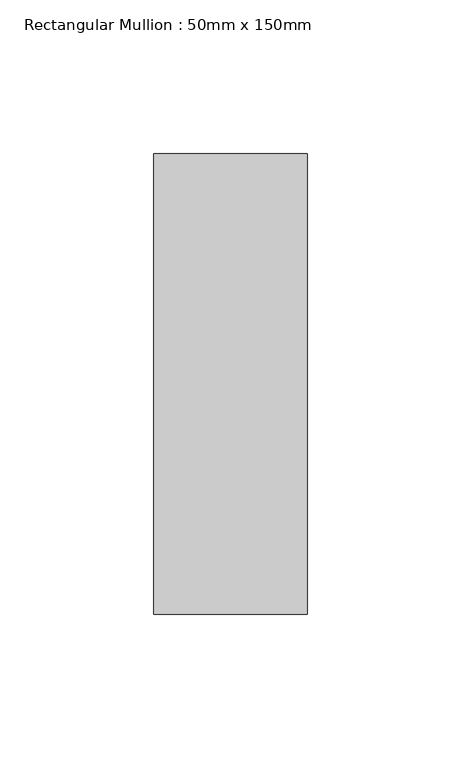
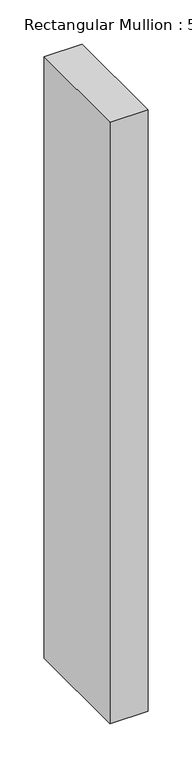
"""IFC4 building model written with IfcOpenShell, lengths in millimetres: member geometry, Rectangular Mullion : 50mm x 150mm."""

from ifc_helpers import new_model, si_unit, frame, origin, place, context, project, spatial, polyline, outline, extrude, source, transform, mapped, element, save


def rectangular_mullion_50mm_x_150mm_e6278944(model_context):
    return source(origin(), model_context, "Body", "SweptSolid", [
        extrude(outline(polyline([(0.0, 75.0), (0.0, -75.0), (-50.0, -75.0), (-50.0, 75.0), (0.0, 75.0)])), frame((0.0, 0.0, -833.3333333), z_axis=(0.0, 0.0, 1.0), x_axis=(1.0, 0.0, 0.0)), (0.0, 0.0, 1.0), 833.3333333),
    ])


if __name__ == "__main__":
    model = new_model("IFC4")
    model_context = context("Model", 3, world=origin())
    ifc_project = project(units=[si_unit("LENGTHUNIT", "METRE", prefix="MILLI")], contexts=[model_context])
    site = spatial("IfcSite", under=ifc_project)
    building = spatial("IfcBuilding", under=site)
    placement = place(None, origin())
    rectangular_mullion_50mm_x_150mm_shape = rectangular_mullion_50mm_x_150mm_e6278944(model_context)
    element("IfcMember", 1, ObjectType="Rectangular Mullion : 50mm x 150mm", at=placement, inside=building, context=model_context, shape_type="MappedRepresentation", body=[
        mapped(rectangular_mullion_50mm_x_150mm_shape, transform((0.0, 0.0, 0.0), x_axis=(1.0, 0.0, 0.0), y_axis=(0.0, 1.0, 0.0), z_axis=(0.0, 0.0, 1.0))),
    ])
    save(model, "model.ifc")

# Revit data of these elements
# Type "Rectangular Mullion : 50mm x 150mm"
#   built-in parameter 1007304 = 0.492126 (stored number, unit not read)
#   built-in parameter 1007301 = 0.082021 (stored number, unit not read)
#   built-in parameter 1007300 = 0.082021 (stored number, unit not read)
# Element 1 (IfcMember, "Rectangular Mullion : 50mm x 150mm")
#   Materials on its faces: "Aluminum"
# Materials
#   "Aluminum": class "Metal", colour RGB 244 244 244, transparency 0, Description = "Aluminum 6061", Cost = 0
